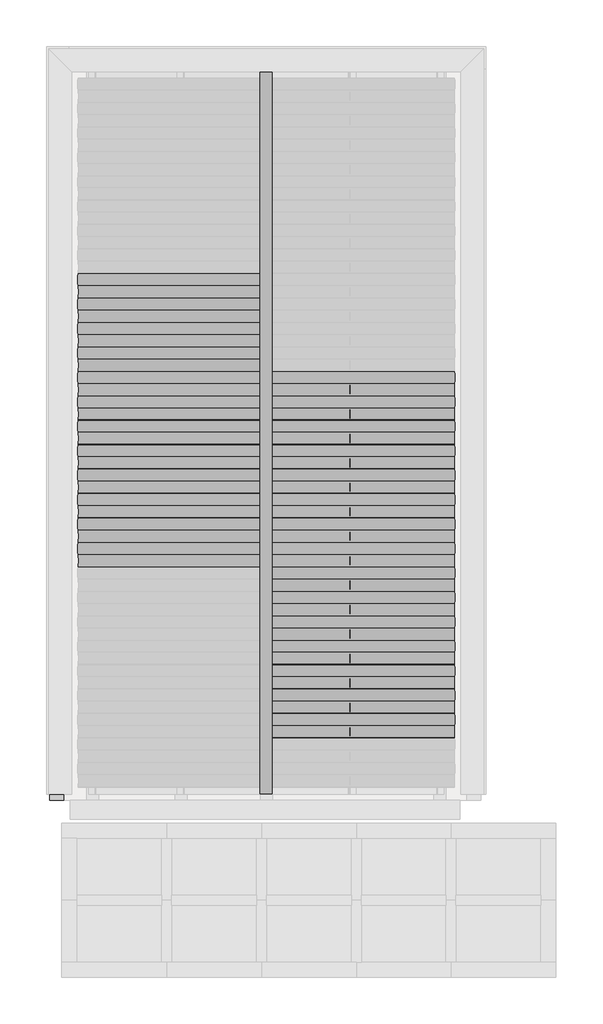
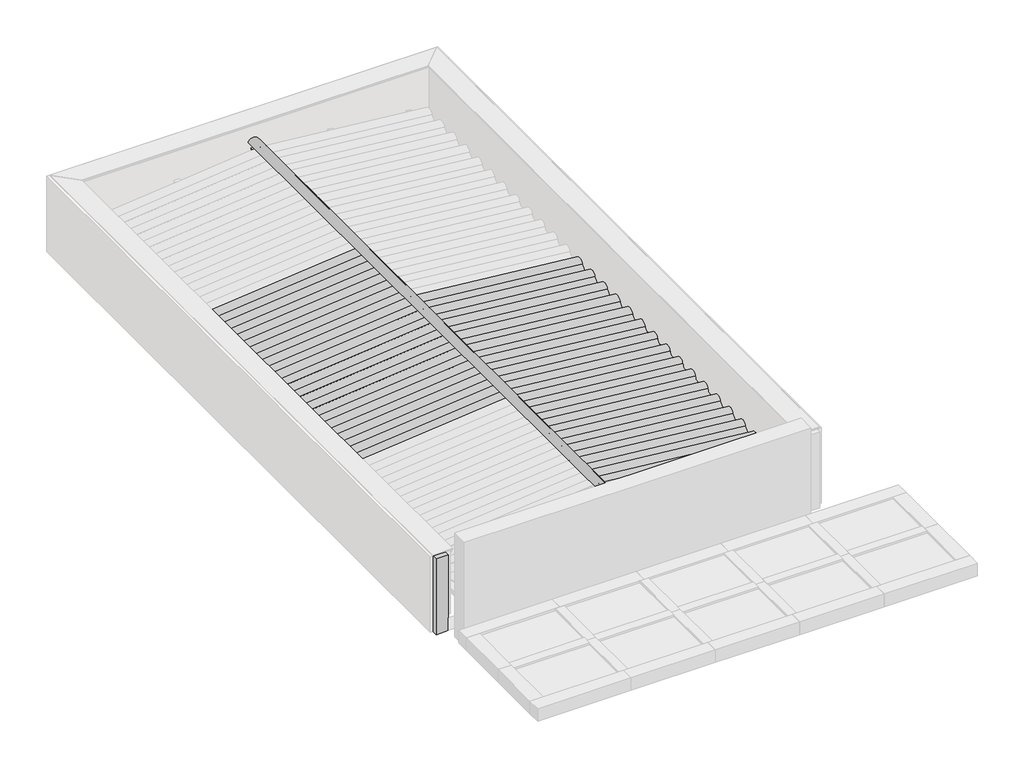
# One storey, part 2 of 3: 35 beams, 6 columns.
# Revit data of these elements (continued)
# Element 6 (IfcBeam, "Cumeeira Telha Ondulada : Fibrocimento") (continued)
#   Phase Created = CC_AP
#   Materials on its faces: ".TELHA DE FIBROCIMENTO"
# Element 7 (IfcBeam, "TQS - Viga retangular : 14.0 x 90.0")
#   Uso = "ESTRUTURA"
#   Titulo = "V103"
#   Chave = "-1269"
#   Tipo Elemento = "Viga"
#   SHA1 = "41485AF0083A76256DE091CB1906E367EBA2D647"
#   Revisão = ""
#   Tipo de carga = ""
#   Divisor de flexao = ""
#   Secao = ""
#   Configuracao = ""
#   Angulo (graus) = ""
#   Detalhamento = ""
#   Casos de vento manual = ""
#   Tipo = ""
#   Alcas = ""
#   Furos = ""
#   Pino = ""
#   Distribuicao = ""
#   Solidarizado = ""
#   Solidarizar na montagem = ""
#   Unir com o próximo = ""
#   Grupo pre moldado = ""
#   Verificado = ""
#   Concreto C = ""
#   Taxa de armadura (kgf/m³) = 0
#   Carga (tf/m²) = 0
#   Carga (tf/m) = 0
#   Carga (tf) = 0
#   Altura = 0.90 m
#   Rebaixo = -0.75 m
#   Largura = 0.14 m
#   Distancia a face = 0.00 m
#   Distancia ao eixo = 0.00 m
#   Altura gerber esquerda = 0.00 m
#   Largura gerber esquerda = 0.00 m
#   Altura gerber direita = 0.00 m
#   Largura gerber direita = 0.00 m
#   Resultado de Ensaios fck (MPa) = 0
#   Unique TQS ID = -1269
#   Principal = yes
#   Structural Material = none
#   Phase Created = CC_PE
# Elements 8, 9, 10, 11, 12, 13, 14, 15, 16, 17, 18, 19, 20, 21, 22, 23, 24, 25, 26, 27, 28, 29, 30, 31, 32, 33, 34 (IfcBeam, "Telha Ondulada : Fibrocimento")
#   Uso = "TELHADOS TELHAS"
#   Phase Created = CC_AP
#   Materials on its faces: ".TELHA DE FIBROCIMENTO"
# Element 35 (IfcBeam, "Madeira de lei : Viga Cumeeira 6x16cm")
#   Comments = ""
#   Uso = "TELHADOS MADEIRAMENTO"
#   Compr Cmcl = 7.50 m
#   Structural Material = .MADEIRAMENTO
#   Phase Created = CC_AP
#   Materials on its faces: ".MADEIRAMENTO"
# Elements 36, 37, 38, 39, 40, 41 (IfcColumn, "Madeira de lei-Coluna : Pontalete 6X16cm")
#   Comments = ""
#   Uso = "TELHADOS ESTRUTURAS"
#   Compr Cmcl = 2.00 m
#   Structural Material = .MADEIRAMENTO
#   Phase Created = CC_AP
#   Materials on its faces: ".MADEIRAMENTO"
# Materials
#   ".TELHA DE FIBROCIMENTO": class "CC_TELHADO", colour RGB 77 77 76, transparency 0, Description = "TELHA ONDULADA FIBROCIMENTO", Cost = 0
#   ".MADEIRAMENTO": class ".CC_MADEIRAS", colour RGB 212 179 113, transparency 0, Cost = 0
# Room, not placed, phase "CC_AP", upper offset 0.00 m, lower offset 0.00 m
#   Number = "31"
#   Name = "Room"
# Room, not placed, phase "CC_AP", upper offset 0.00 m, lower offset 0.00 m
#   Number = "34"
#   Name = "Room"
